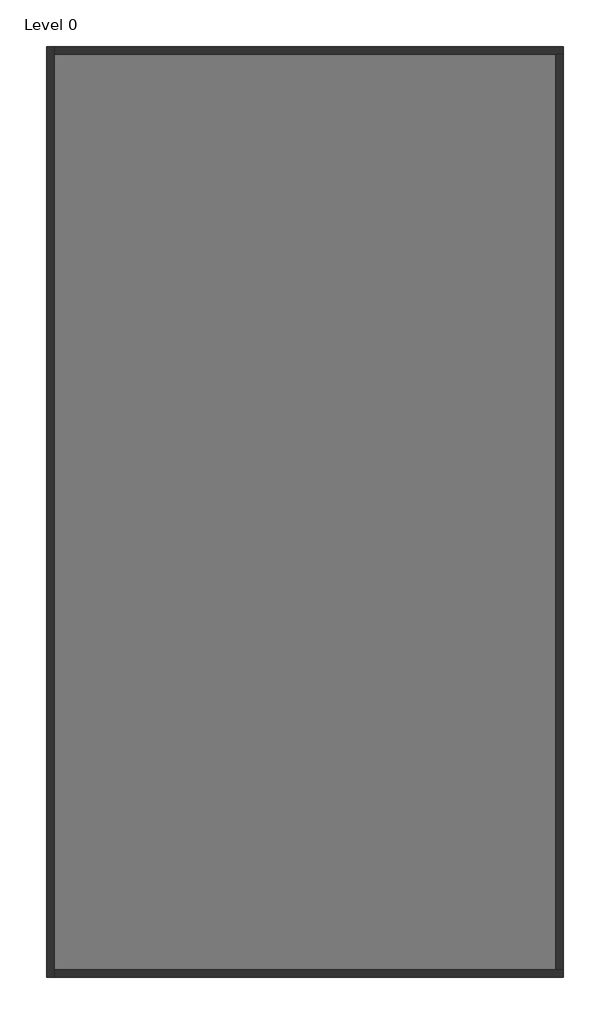
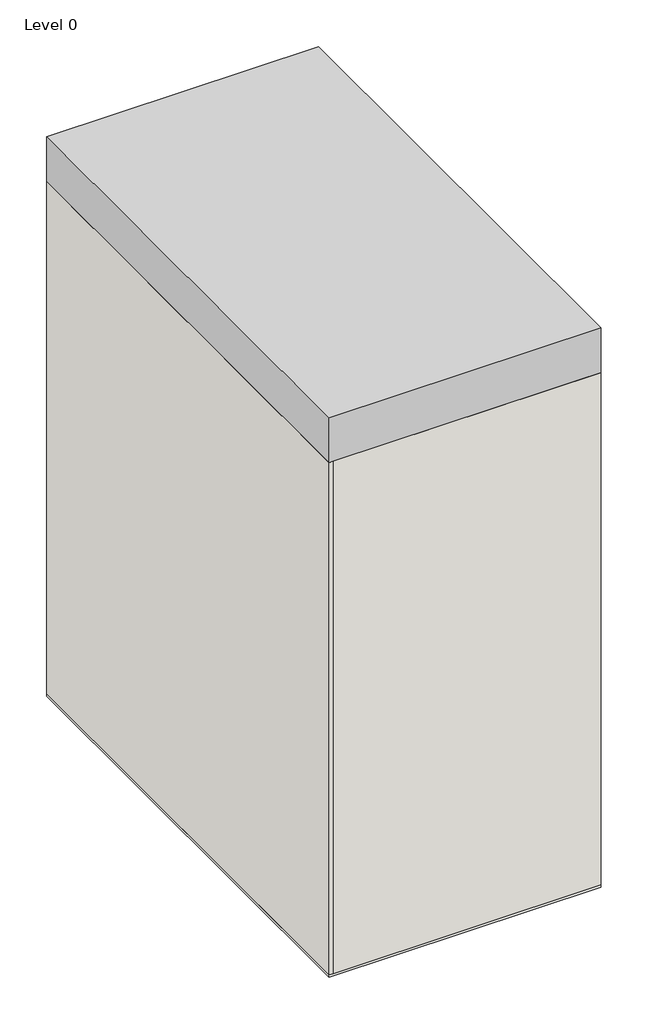
# One storey: 4 walls, 1 proxy, 1 slab.
"""IFC4 building model written with IfcOpenShell, lengths in millimetres."""

from ifc_helpers import new_model, si_unit, frame, origin, origin_with_axes, place, context, project, spatial, polyline, outline, extrude, faceted_brep, element, save

model = new_model("IFC4")

# Units and contexts
model_context = context("Model", 3, world=origin())
ifc_project = project(units=[si_unit("LENGTHUNIT", "METRE", prefix="MILLI")], contexts=[model_context])

# Site, building, storey
site = spatial("IfcSite", under=ifc_project)
building = spatial("IfcBuilding", under=site)
storey = spatial("IfcBuildingStorey", under=building, Name="Level 0", Elevation=100.0)

# Proxy
placement = place(None, origin())
element("IfcBuildingElementProxy", 1, Name="LowUrbanDensityBuilding : LowUrbanDensityBuilding", ObjectType="LowUrbanDensityBuilding : LowUrbanDensityBuilding", at=placement, inside=storey, context=model_context, shape_type="SweptSolid", body=[
    extrude(outline(polyline([(7325.2659446, 3676.2074539), (7325.2659446, -14323.7925461), (-2674.7340554, -14323.7925461), (-2674.7340554, 3676.2074539), (7325.2659446, 3676.2074539)])), origin_with_axes(), (0.0, 0.0, 1.0), 21749.8),
])

# Slab
element("IfcSlab", 2, ObjectType="Floor-Concrete_100Con", at=placement, inside=storey, context=model_context, shape_type="SweptSolid", body=[
    extrude(outline(polyline([(7325.2659446, 3676.2074539), (7325.2659446, -14323.7925461), (-2674.7340554, -14323.7925461), (-2674.7340554, 3676.2074539), (7325.2659446, 3676.2074539)])), origin_with_axes(), (0.0, 0.0, 1.0), 100.0),
])

# Walls
element("IfcWall", 3, ObjectType="Wall-Ext_25Rdr-100Blk-19P", at=placement, inside=storey, context=model_context, shape_type="Brep", body=[
    faceted_brep([(-2674.7340554, 3676.2074539, 100.0), (-2674.7340554, -14323.7925461, 100.0), (-2674.7340554, -14323.7925461, 20000.0), (-2674.7340554, 3676.2074539, 20000.0), (-2530.4340554, 3676.2074539, 100.0), (-2530.4340554, 3676.2074539, 20000.0), (-2530.4340554, 3531.9074539, 20000.0), (-2530.4340554, -14179.4925461, 20000.0), (-2530.4340554, -14323.7925461, 20000.0), (-2530.4340554, -14323.7925461, 100.0), (-2530.4340554, -14179.4925461, 100.0), (-2530.4340554, 3531.9074539, 100.0)], [[[0, 1, 2, 3]], [[4, 5, 6, 7, 8, 9, 10, 11]], [[1, 0, 4, 11, 10, 9]], [[3, 2, 8, 7, 6, 5]], [[2, 1, 9, 8]], [[0, 3, 5, 4]]]),
])
element("IfcWall", 4, ObjectType="Wall-Ext_25Rdr-100Blk-19P", at=placement, inside=storey, context=model_context, shape_type="Brep", body=[
    faceted_brep([(-2530.4340554, -14323.7925461, 100.0), (7325.2659446, -14323.7925461, 100.0), (7325.2659446, -14323.7925461, 20000.0), (-2530.4340554, -14323.7925461, 20000.0), (-2530.4340554, -14179.4925461, 100.0), (-2530.4340554, -14179.4925461, 20000.0), (7180.9659446, -14179.4925461, 20000.0), (7325.2659446, -14179.4925461, 20000.0), (7325.2659446, -14179.4925461, 100.0), (7180.9659446, -14179.4925461, 100.0)], [[[0, 1, 2, 3]], [[4, 5, 6, 7, 8, 9]], [[1, 0, 4, 9, 8]], [[3, 2, 7, 6, 5]], [[0, 3, 5, 4]], [[2, 1, 8, 7]]]),
])
element("IfcWall", 5, ObjectType="Wall-Ext_25Rdr-100Blk-19P", at=placement, inside=storey, context=model_context, shape_type="Brep", body=[
    faceted_brep([(7325.2659446, 3676.2074539, 100.0), (-2530.4340554, 3676.2074539, 100.0), (-2530.4340554, 3676.2074539, 20000.0), (7325.2659446, 3676.2074539, 20000.0), (7325.2659446, 3531.9074539, 100.0), (7325.2659446, 3531.9074539, 20000.0), (7180.9659446, 3531.9074539, 20000.0), (-2530.4340554, 3531.9074539, 20000.0), (-2530.4340554, 3531.9074539, 100.0), (7180.9659446, 3531.9074539, 100.0)], [[[0, 1, 2, 3]], [[4, 5, 6, 7, 8, 9]], [[1, 0, 4, 9, 8]], [[3, 2, 7, 6, 5]], [[2, 1, 8, 7]], [[0, 3, 5, 4]]]),
])
element("IfcWall", 6, ObjectType="Wall-Ext_25Rdr-100Blk-19P", at=placement, inside=storey, context=model_context, shape_type="SweptSolid", body=[
    extrude(outline(polyline([(7325.2659446, 3531.9074539), (7325.2659446, -14179.4925461), (7180.9659446, -14179.4925461), (7180.9659446, 3531.9074539), (7325.2659446, 3531.9074539)])), frame((0.0, 0.0, 100.0), z_axis=(0.0, 0.0, 1.0), x_axis=(1.0, 0.0, 0.0)), (0.0, 0.0, 1.0), 19900.0),
])

save(model, "model.ifc")

# Revit data of these elements
# Project information
#   Project Issue Date = "Issue Date"
#   Project Status = "Project Status"
#   Client Name = "Owner"
#   Project Address = "Enter address here"
#   Project Name = "Project Name"
#   Project Number = "Project Number"
# Type "Floor-Concrete_100Con"
#   Keynote = "E60/130"
#   Function = 0
#   Layers, outside or top first: 100 mm "Concrete" (function 1)
# Type "Wall-Ext_25Rdr-100Blk-19P"
#   Keynote = "F10"
#   Layers, outside or top first: 25.3 mm "Render, Beige, Smooth" (function 5); 100 mm "Concrete Masonry Units _Low Density" (function 1); 19 mm "Plaster" (function 5)
# Element 1 (IfcBuildingElementProxy, "LowUrbanDensityBuilding : LowUrbanDensityBuilding")
#   Phase Created = New Construction
#   Materials on its faces: "Default Form"
# Element 2 (IfcSlab, "Floor-Concrete_100Con")
#   Height Offset From Level = 0 mm
#   Phase Created = New Construction
#   Materials on its faces: "Concrete"
# Element 3 (IfcWall, "Wall-Ext_25Rdr-100Blk-19P")
#   Top Offset = 0 mm
#   Base Offset = 0 mm
#   wall height = 19900 mm
#   Phase Created = New Construction
#   Base Constraint = Level 0
#   Top Constraint = Level 5
#   Materials on its faces: "Render, Beige, Smooth", "Default Wall", "Plaster"
# Elements 4, 5, 6 (IfcWall, "Wall-Ext_25Rdr-100Blk-19P")
#   Top Offset = 0 mm
#   Base Offset = 0 mm
#   wall height = 19900 mm
#   Phase Created = New Construction
#   Base Constraint = Level 0
#   Top Constraint = Level 5
#   Materials on its faces: "Default Wall", "Render, Beige, Smooth", "Plaster"
# Materials
#   "Concrete": class "Concrete", colour RGB 120 120 120, transparency 0, Description = "Portland Cement Concrete", Cost = 0
#   "Render, Beige, Smooth": class "Generic", colour RGB 213 198 180, transparency 0, Description = "physical material", Cost = 0
#   "Concrete Masonry Units _Low Density": class "Masonry", colour RGB 181 181 181, transparency 0, Description = "Concrete masonry units", Cost = 0
#   "Plaster": class "Generic", colour RGB 249 249 249, transparency 0, Description = "Plaster", Cost = 0
#   "Default Form": class "Generic", colour RGB 185 189 196, transparency 0.5, Cost = 0
#   "Default Wall": class "Miscellaneous", colour RGB 128 128 128, transparency 0, Comments = "Rendering appearance not upgraded Rendering appearance not upgraded ", Cost = 0
